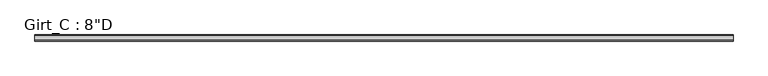
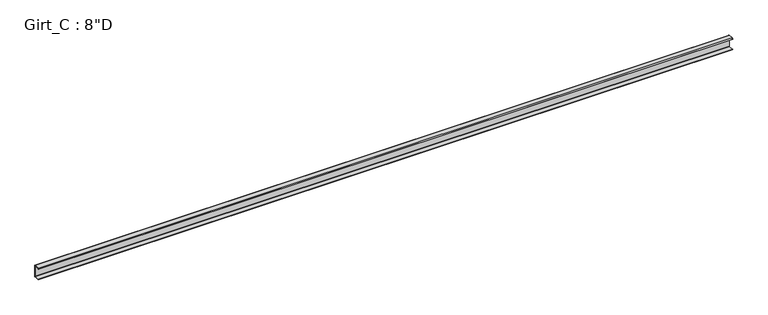
"""IFC4 building model written with IfcOpenShell, lengths in millimetres: beam geometry."""

import ifcopenshell
import ifcopenshell.guid

model = None  # the IFC model being written
_history = None  # IfcOwnerHistory: only IFC2X3 demands one
_inside = {}  # id of a spatial element -> (the spatial element, [elements in it])
_under = {}  # id of a project, library or spatial element -> (it, [spatial elements below it])
_declared = {}  # id of a project -> (the project, [libraries it declares])
_typed = {}  # id of a type object -> (the type object, [elements of that type])
_made_of = {}  # id of a material, layer set ... -> (it, [elements and type objects made of it])


def new_model(schema):
    """Start an empty IFC model of exactly this schema.

    Asked for "IFC4X3", IfcOpenShell would pick the latest addendum, in which some entities
    have other attributes; the version numbers below select the first issue.
    IFC2X3 requires an IfcOwnerHistory on every rooted entity: one is made here for all.
    """
    global model, _history
    if schema == "IFC4X3":
        model = ifcopenshell.file(schema_version=(4, 3, 0, 0))
    else:
        model = ifcopenshell.file(schema=schema)
    _inside.clear()
    _under.clear()
    _declared.clear()
    _typed.clear()
    _made_of.clear()
    _history = None
    if model.schema == "IFC2X3":
        org = make("IfcOrganization", Name="unknown")
        user = make(
            "IfcPersonAndOrganization",
            ThePerson=make("IfcPerson", FamilyName="unknown"),
            TheOrganization=org,
        )
        app = make(
            "IfcApplication",
            ApplicationDeveloper=org,
            Version="unknown",
            ApplicationFullName="unknown",
            ApplicationIdentifier="unknown",
        )
        _history = make(
            "IfcOwnerHistory",
            OwningUser=user,
            OwningApplication=app,
            ChangeAction="ADDED",
            CreationDate=0,
        )
    return model


def make(cls, **values):
    """One entity of the class cls with the attributes given. An attribute that is None is left unset."""
    return model.create_entity(
        cls, **{name: value for name, value in values.items() if value is not None}
    )


def rooted(cls, **values):
    """An entity with a GlobalId (a new one), such as an element, a storey or a relation."""
    return make(cls, GlobalId=ifcopenshell.guid.new(), OwnerHistory=_history, **values)


def si_unit(unit_type, name, prefix=None):
    """IfcSIUnit, for example si_unit("LENGTHUNIT", "METRE", prefix="MILLI")."""
    return make("IfcSIUnit", UnitType=unit_type, Prefix=prefix, Name=name)


def assignment(units):
    """IfcUnitAssignment: the units of a project."""
    return None if units is None else make("IfcUnitAssignment", Units=units)


def point(xyz):
    """IfcCartesianPoint."""
    return None if xyz is None else make("IfcCartesianPoint", Coordinates=xyz)


def direction(xyz):
    """IfcDirection."""
    return None if xyz is None else make("IfcDirection", DirectionRatios=xyz)


def frame(location, z_axis=None, x_axis=None):
    """IfcAxis2Placement3D, a coordinate frame: its origin and axes. An axis left out is left unset."""
    return make(
        "IfcAxis2Placement3D",
        Location=point(location),
        Axis=direction(z_axis),
        RefDirection=direction(x_axis),
    )


def frame_2d(location, x_axis=None):
    """IfcAxis2Placement2D, a coordinate frame in the plane: its origin and x axis."""
    return make(
        "IfcAxis2Placement2D", Location=point(location), RefDirection=direction(x_axis)
    )


def origin():
    """The frame at (0, 0, 0) with its axes left unset."""
    return frame((0.0, 0.0, 0.0))


def place(relative_to, where):
    """IfcLocalPlacement: puts the frame where relative to a parent placement (None: the world)."""
    return make(
        "IfcLocalPlacement", PlacementRelTo=relative_to, RelativePlacement=where
    )


def context(
    kind, dimensions, precision=None, world=None, true_north=None, identifier=None
):
    """IfcGeometricRepresentationContext, for example the 3D "Model" context."""
    return make(
        "IfcGeometricRepresentationContext",
        ContextIdentifier=identifier,
        ContextType=kind,
        CoordinateSpaceDimension=dimensions,
        Precision=precision,
        WorldCoordinateSystem=world,
        TrueNorth=true_north,
    )


def project(units=None, contexts=None):
    """IfcProject with its units and contexts."""
    return rooted(
        "IfcProject",
        Name="project",
        RepresentationContexts=contexts,
        UnitsInContext=assignment(units),
    )


def spatial(cls, under=None, at=None, **own):
    """A site, building, storey or space (cls), placed at a placement, below another one or the project."""
    s = rooted(cls, ObjectPlacement=at, **own)
    if under is not None:
        _under.setdefault(under.id(), (under, []))[1].append(s)
    return s


def polyline(points):
    """IfcPolyline through the points."""
    return make("IfcPolyline", Points=[point(p) for p in points])


def circle_curve(where, radius):
    """IfcCircle in the frame where."""
    return make("IfcCircle", Position=where, Radius=radius)


def trimmed(basis, trim1, trim2, sense, master):
    """IfcTrimmedCurve: the piece of a basis curve between two trims."""
    return make(
        "IfcTrimmedCurve",
        BasisCurve=basis,
        Trim1=trim1,
        Trim2=trim2,
        SenseAgreement=sense,
        MasterRepresentation=master,
    )


def segment(curve, same_sense, transition):
    """IfcCompositeCurveSegment."""
    return make(
        "IfcCompositeCurveSegment",
        Transition=transition,
        SameSense=same_sense,
        ParentCurve=curve,
    )


def composite_curve(segments, self_intersect=None):
    """IfcCompositeCurve: segments joined end to end."""
    return make("IfcCompositeCurve", Segments=segments, SelfIntersect=self_intersect)


def outline(outer, holes=None, kind="AREA"):
    """IfcArbitraryClosedProfileDef: a profile drawn as a closed curve; with holes, ...WithVoids."""
    if holes is None:
        return make("IfcArbitraryClosedProfileDef", ProfileType=kind, OuterCurve=outer)
    return make(
        "IfcArbitraryProfileDefWithVoids",
        ProfileType=kind,
        OuterCurve=outer,
        InnerCurves=holes,
    )


def extrude(swept, where, along, depth):
    """IfcExtrudedAreaSolid: the profile swept, set in the frame where, extruded along a direction by depth."""
    return make(
        "IfcExtrudedAreaSolid",
        SweptArea=swept,
        Position=where,
        ExtrudedDirection=direction(along),
        Depth=depth,
    )


def shape(context_of_items, identifier, shape_type, items):
    """IfcShapeRepresentation: the items that make up one representation, for example the "Body"."""
    return make(
        "IfcShapeRepresentation",
        ContextOfItems=context_of_items,
        RepresentationIdentifier=identifier,
        RepresentationType=shape_type,
        Items=items,
    )


def source(mapping_origin, context_of_items, identifier, shape_type, items):
    """IfcRepresentationMap: a shape defined once, which mapped items show again and again."""
    return make(
        "IfcRepresentationMap",
        MappingOrigin=mapping_origin,
        MappedRepresentation=shape(context_of_items, identifier, shape_type, items),
    )


def transform(
    local_origin,
    x_axis=None,
    y_axis=None,
    z_axis=None,
    scale=None,
    scale2=None,
    scale3=None,
    uniform=True,
):
    """IfcCartesianTransformationOperator3D, or its non-uniform kind. x_axis, y_axis, z_axis: its Axis1, 2, 3."""
    if uniform:
        return make(
            "IfcCartesianTransformationOperator3D",
            Axis1=direction(x_axis),
            Axis2=direction(y_axis),
            LocalOrigin=point(local_origin),
            Scale=scale,
            Axis3=direction(z_axis),
        )
    return make(
        "IfcCartesianTransformationOperator3DnonUniform",
        Axis1=direction(x_axis),
        Axis2=direction(y_axis),
        LocalOrigin=point(local_origin),
        Scale=scale,
        Axis3=direction(z_axis),
        Scale2=scale2,
        Scale3=scale3,
    )


def mapped(mapping_source, mapping_target):
    """IfcMappedItem: shows the shape of a source again, moved by a transform."""
    return make(
        "IfcMappedItem", MappingSource=mapping_source, MappingTarget=mapping_target
    )


def made_of(thing, what):
    """Note that an element or type object is made of a material, layer set ...; save() writes the relation."""
    if what is not None:
        _made_of.setdefault(what.id(), (what, []))[1].append(thing)
    return thing


def element(
    cls,
    number,
    at=None,
    inside=None,
    cuts=None,
    type_object=None,
    material=None,
    context=None,
    identifier="Body",
    shape_type=None,
    held_by="IfcProductDefinitionShape",
    body=None,
    shapes=None,
    **own,
):
    """One element of the class cls, such as IfcWall. Its Tag is "e" and its number.

    at: its placement. inside: the storey or other place that contains it. cuts: it is an
    opening in that element (IfcRelVoidsElement). A single representation is given by context,
    identifier, shape_type and body (its items); several are given by shapes. held_by: the class
    of the entity that holds the representations. save() writes the other relations.
    """
    e = rooted(cls, Tag="e%d" % number, ObjectPlacement=at, **own)
    if body is not None:
        shapes = [shape(context, identifier, shape_type, body)]
    if shapes is not None:
        e.Representation = make(held_by, Representations=shapes)
    if inside is not None:
        _inside.setdefault(inside.id(), (inside, []))[1].append(e)
    if cuts is not None:
        rooted(
            "IfcRelVoidsElement", RelatingBuildingElement=cuts, RelatedOpeningElement=e
        )
    if type_object is not None:
        _typed.setdefault(type_object.id(), (type_object, []))[1].append(e)
    return made_of(e, material)


def aggregate(whole, parts):
    """IfcRelAggregates: a whole, such as a stair, and the parts it consists of."""
    return rooted("IfcRelAggregates", RelatingObject=whole, RelatedObjects=parts)


def save(model, path):
    """Write the relations noted so far, then the file.

    IfcRelAggregates (storeys below a building ...), IfcRelContainedInSpatialStructure (elements
    in a storey), IfcRelDefinesByType, IfcRelAssociatesMaterial and IfcRelDeclares: one each for
    every whole, place, type object, material and project.
    """
    for whole, parts in _under.values():
        aggregate(whole, parts)
    for where, things in _inside.values():
        rooted(
            "IfcRelContainedInSpatialStructure",
            RelatedElements=things,
            RelatingStructure=where,
        )
    for kind, things in _typed.values():
        rooted("IfcRelDefinesByType", RelatedObjects=things, RelatingType=kind)
    for what, things in _made_of.values():
        rooted("IfcRelAssociatesMaterial", RelatedObjects=things, RelatingMaterial=what)
    for by, libraries in _declared.values():
        rooted("IfcRelDeclares", RelatingContext=by, RelatedDefinitions=libraries)
    model.write(path)


def beam_ac5e974c(model_context):
    return source(origin(), model_context, "Body", "SweptSolid", [
        extrude(outline(composite_curve([segment(polyline([(-87.5109375, 101.6), (-3.3734375, 101.6)]), True, "CONTINUOUS"), segment(trimmed(circle_curve(frame_2d((-3.3734375, 96.8375)), 4.7625), [point((-3.3734375, 101.6))], [point((1.3890625, 96.8375))], False, "CARTESIAN"), True, "CONTINUOUS"), segment(polyline([(1.3890625, 96.8375), (1.3890625, -96.8375)]), True, "CONTINUOUS"), segment(trimmed(circle_curve(frame_2d((-3.3734375, -96.8375)), 4.7625), [point((1.3890625, -96.8375))], [point((-3.3734375, -101.6))], False, "CARTESIAN"), True, "CONTINUOUS"), segment(polyline([(-3.3734375, -101.6), (-87.5109375, -101.6), (-99.7792647, -86.979177), (-97.6510975, -85.1934327), (-86.2154765, -98.821875), (-3.2694106, -98.821875)]), True, "CONTINUOUS"), segment(trimmed(circle_curve(frame_2d((-3.3748024, -96.8389339)), 1.9857399), [point((-3.2694106, -98.821875))], [point((-1.3890625, -96.8389339))], True, "CARTESIAN"), True, "CONTINUOUS"), segment(polyline([(-1.3890625, -96.8389339), (-1.3890625, 96.8381931)]), True, "CONTINUOUS"), segment(trimmed(circle_curve(frame_2d((-3.3741066, 96.8381931)), 1.9850441), [point((-1.3890625, 96.8381931))], [point((-3.3005807, 98.821875))], True, "CARTESIAN"), True, "CONTINUOUS"), segment(polyline([(-3.3005807, 98.821875), (-86.2154765, 98.821875), (-97.6278742, 85.221109), (-99.7560415, 87.0068534), (-87.5109375, 101.6)]), True, "CONTINUOUS")], self_intersect=False)), frame((-5735.1929994, 0.0, 0.0), z_axis=(1.0, 0.0, 0.0), x_axis=(0.0, 1.0, 0.0)), (0.0, 0.0, 1.0), 11489.6955156),
    ])


if __name__ == "__main__":
    model = new_model("IFC4")
    model_context = context("Model", 3, world=origin())
    ifc_project = project(units=[si_unit("LENGTHUNIT", "METRE", prefix="MILLI")], contexts=[model_context])
    site = spatial("IfcSite", under=ifc_project)
    building = spatial("IfcBuilding", under=site)
    placement = place(None, origin())
    beam_shape = beam_ac5e974c(model_context)
    element("IfcBeam", 1, ObjectType="Girt_C : 8\"D", at=placement, inside=building, context=model_context, shape_type="MappedRepresentation", body=[
        mapped(beam_shape, transform((0.0, 0.0, 0.0), x_axis=(1.0, 0.0, 0.0), y_axis=(0.0, 1.0, 0.0), z_axis=(0.0, 0.0, 1.0))),
    ])
    save(model, "model.ifc")

# Revit data of these elements
# Type "Girt_C : 8\"D"
#   half leg = 0' - 1 3/4"
#   Web_Thickness = 0' - 0 7/64"
#   Length [instance default] = 10' - 0"
#   Leg_1 = 0' - 3 1/2"
#   Height = 0' - 8"
#   Structural Material [instance default] = none
# Element 1 (IfcBeam, "Girt_C : 8\"D")
#   Structural Material = GALVANIZED 'CEE' SECTION (8.0x3.5C - SEE STRUCT. DWGS)
#   Materials on its faces: "GALVANIZED 'CEE' SECTION (8.0x3.5C - SEE STRUCT. DWGS)"
# Materials
#   "GALVANIZED 'CEE' SECTION (8.0x3.5C - SEE STRUCT. DWGS)": class "Metal", colour RGB 137 146 153, transparency 0, Description = "Steel, mill finish", Cost = 0
